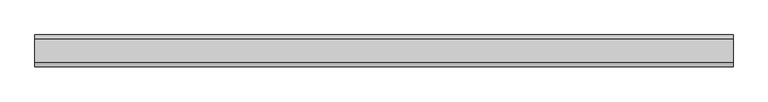
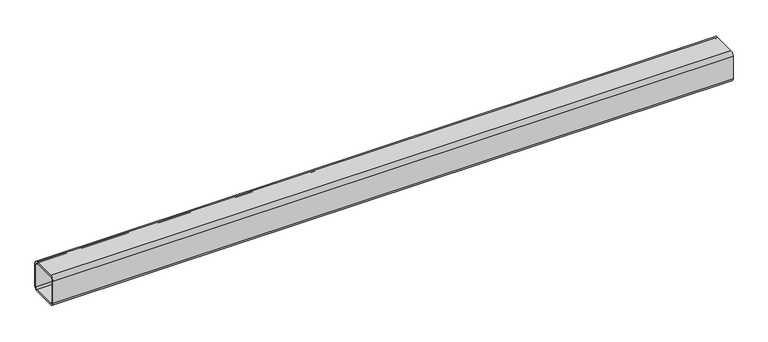
"""IFC4 building model written with IfcOpenShell, lengths in millimetres: beam geometry, Гнутый прямоугольный профиль (Трубы 30245-94) Балки : гнутый прямоуг. проф. 100x6."""

from ifc_helpers import new_model, si_unit, point, frame, frame_2d, origin, place, context, project, spatial, polyline, circle_curve, trimmed, segment, composite_curve, outline, extrude, source, transform, mapped, element, save


def beam_71c8164e(model_context):
    return source(origin(), model_context, "Body", "SweptSolid", [
        extrude(outline(composite_curve([segment(polyline([(-38.0, 50.0), (38.0, 50.0)]), True, "CONTINUOUS"), segment(trimmed(circle_curve(frame_2d((38.0, 38.0)), 12.0), [point((38.0, 50.0))], [point((50.0, 38.0))], False, "CARTESIAN"), True, "CONTINUOUS"), segment(polyline([(50.0, 38.0), (50.0, -38.0)]), True, "CONTINUOUS"), segment(trimmed(circle_curve(frame_2d((38.0, -38.0)), 12.0), [point((50.0, -38.0))], [point((38.0, -50.0))], False, "CARTESIAN"), True, "CONTINUOUS"), segment(polyline([(38.0, -50.0), (-38.0, -50.0)]), True, "CONTINUOUS"), segment(trimmed(circle_curve(frame_2d((-38.0, -38.0)), 12.0), [point((-38.0, -50.0))], [point((-50.0, -38.0))], False, "CARTESIAN"), True, "CONTINUOUS"), segment(polyline([(-50.0, -38.0), (-50.0, 38.0)]), True, "CONTINUOUS"), segment(trimmed(circle_curve(frame_2d((-38.0, 38.0)), 12.0), [point((-50.0, 38.0))], [point((-38.0, 50.0))], False, "CARTESIAN"), True, "CONTINUOUS")], self_intersect=False), holes=[composite_curve([segment(trimmed(circle_curve(frame_2d((-38.0, 38.0)), 6.0), [point((-38.0, 44.0))], [point((-44.0, 38.0))], True, "CARTESIAN"), True, "CONTINUOUS"), segment(polyline([(-44.0, 38.0), (-44.0, -38.0)]), True, "CONTINUOUS"), segment(trimmed(circle_curve(frame_2d((-38.0, -38.0)), 6.0), [point((-44.0, -38.0))], [point((-38.0, -44.0))], True, "CARTESIAN"), True, "CONTINUOUS"), segment(polyline([(-38.0, -44.0), (38.0, -44.0)]), True, "CONTINUOUS"), segment(trimmed(circle_curve(frame_2d((38.0, -38.0)), 6.0), [point((38.0, -44.0))], [point((44.0, -38.0))], True, "CARTESIAN"), True, "CONTINUOUS"), segment(polyline([(44.0, -38.0), (44.0, 38.0)]), True, "CONTINUOUS"), segment(trimmed(circle_curve(frame_2d((38.0, 38.0)), 6.0), [point((44.0, 38.0))], [point((38.0, 44.0))], True, "CARTESIAN"), True, "CONTINUOUS"), segment(polyline([(38.0, 44.0), (-38.0, 44.0)]), True, "CONTINUOUS")], self_intersect=False)]), frame((-1094.5, 0.0, 0.0), z_axis=(1.0, 0.0, 0.0), x_axis=(0.0, 1.0, 0.0)), (0.0, 0.0, 1.0), 2189.0),
    ])


if __name__ == "__main__":
    model = new_model("IFC4")
    model_context = context("Model", 3, world=origin())
    ifc_project = project(units=[si_unit("LENGTHUNIT", "METRE", prefix="MILLI")], contexts=[model_context])
    site = spatial("IfcSite", under=ifc_project)
    building = spatial("IfcBuilding", under=site)
    placement = place(None, origin())
    beam_shape = beam_71c8164e(model_context)
    element("IfcBeam", 1, ObjectType="Гнутый прямоугольный профиль (Трубы 30245-94) Балки : гнутый прямоуг. проф. 100x6", at=placement, inside=building, context=model_context, shape_type="MappedRepresentation", body=[
        mapped(beam_shape, transform((0.0, 0.0, 0.0), x_axis=(1.0, 0.0, 0.0), y_axis=(0.0, 1.0, 0.0), z_axis=(0.0, 0.0, 1.0))),
    ])
    save(model, "model.ifc")

# Revit data of these elements
# Type "Гнутый прямоугольный профиль (Трубы 30245-94) Балки : гнутый прямоуг. проф. 100x6"
#   ri = 12 mm
#   ra = 6 mm
#   W = 0.173578
#   Vz = 50 mm
#   Vy = 50 mm
#   Vpz = 50 mm
#   Vpy = 50 mm
#   Length [instance default] = 1500 mm
#   bf = 100 mm
#   d = 100 mm
#   tf = 6 mm
#   tw = 6 mm
#   A = 0.00226 m²
#   Structural Material [instance default] = Металл - Сталь - 345 МПa
#   Assembly Code = ""
# Element 1 (IfcBeam, "Гнутый прямоугольный профиль (Трубы 30245-94) Балки : гнутый прямоуг. проф. 100x6")
#   Structural Material = C235
#   Materials on its faces: "C235"
# Materials
#   "Металл - Сталь - 345 МПa": class "Металл", colour RGB 247 247 247, transparency 0
#   "C235": class "Не назначено", colour RGB 0 0 0, transparency 0
